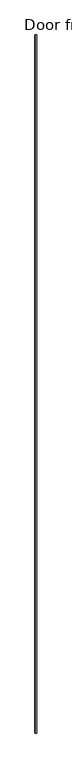
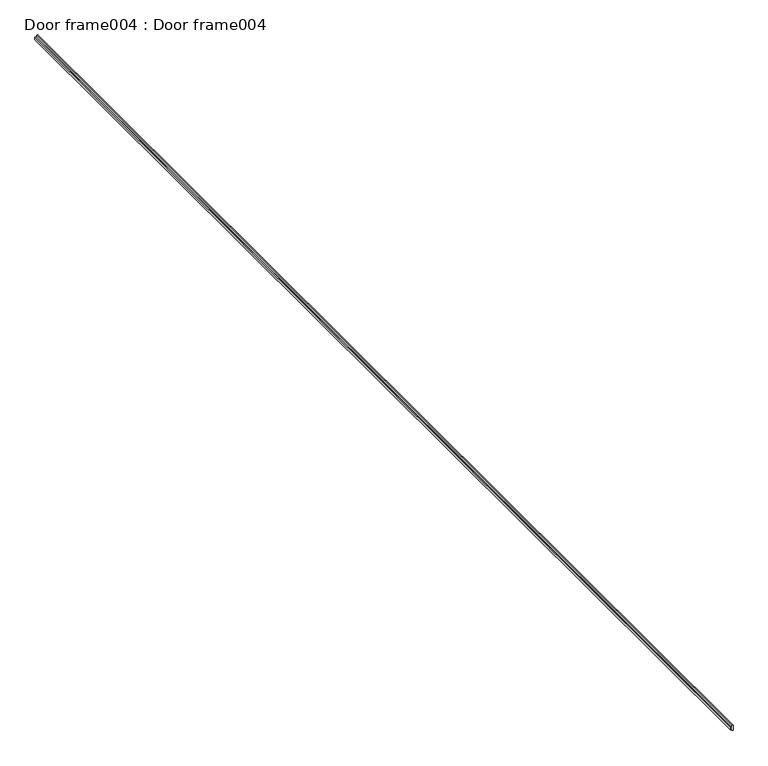
"""IFC4 building model written with IfcOpenShell, lengths in millimetres: proxy geometry, Door frame004 : Door frame004."""

from ifc_helpers import new_model, si_unit, frame, origin, place, context, project, spatial, polyline, outline, extrude, source, transform, mapped, element, save


def door_frame004_door_frame004_03d84ab6(model_context):
    return source(origin(), model_context, "Body", "SweptSolid", [
        extrude(outline(polyline([(36685.3750947, 15525.9592515), (36685.3750947, 15524.8924515), (36680.8030947, 15524.8924515), (36680.8030947, 15525.9592515), (36682.2000947, 15525.9592515), (36682.2000947, 15527.7372515), (36678.7014343, 15527.7372515), (36678.7014343, 15529.9292246), (36687.4772673, 15529.9292246), (36687.4772673, 15527.7373022), (36683.9780947, 15527.7373022), (36683.9780947, 15525.9592515), (36685.3750947, 15525.9592515)])), frame((0.0, -1052.8906567, 0.0), z_axis=(0.0, 1.0, 0.0), x_axis=(0.0, 0.0, 1.0)), (0.0, 0.0, 1.0), 1999.85),
    ])


if __name__ == "__main__":
    model = new_model("IFC4")
    model_context = context("Model", 3, world=origin())
    ifc_project = project(units=[si_unit("LENGTHUNIT", "METRE", prefix="MILLI")], contexts=[model_context])
    site = spatial("IfcSite", under=ifc_project)
    building = spatial("IfcBuilding", under=site)
    placement = place(None, origin())
    door_frame004_door_frame004_shape = door_frame004_door_frame004_03d84ab6(model_context)
    element("IfcBuildingElementProxy", 1, Name="Door frame004 : Door frame004", ObjectType="Door frame004 : Door frame004", at=placement, inside=building, context=model_context, shape_type="MappedRepresentation", body=[
        mapped(door_frame004_door_frame004_shape, transform((0.0, 0.0, 0.0), x_axis=(1.0, 0.0, 0.0), y_axis=(0.0, 1.0, 0.0), z_axis=(0.0, 0.0, 1.0))),
    ])
    save(model, "model.ifc")

# Revit data of these elements
# Project information
#   Issued Date 1 = "0/00/2018 - City of Newport Beach"
#   IfcSite GUID = "3hCLsSIbaHwOLX093rt3ko"
#   IfcBuilding GUID = "3hCN2YIbaHwOLX093rt3ko"
#   IfcProject GUID = "7043067b_ee86_4e71_a94"
#   NameOverride = "Default Site"
#   Project Issue Date = "Issue Date"
#   Project Status = "Project Status"
#   Client Name = "xxx"
#   Project Address = "xxx"
#   Project Name = "STAUDENMEIER RESIDENCE"
# Type "Door frame004 : Door frame004"
#   NameOverride = "Door frame004"
# Element 1 (IfcBuildingElementProxy, "Door frame004 : Door frame004")
#   Materials on its faces: "FLEETWOOD SERIES T-3200 SINGLE SWING DOOR FRAME"
# Materials
#   "FLEETWOOD SERIES T-3200 SINGLE SWING DOOR FRAME": class "Unassigned", colour RGB 128 128 128, transparency 0, Cost = 0
